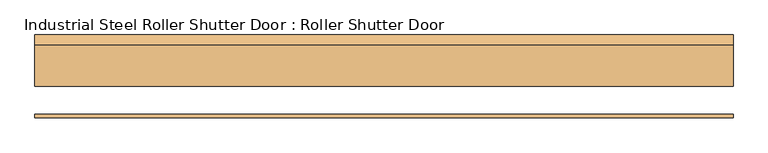
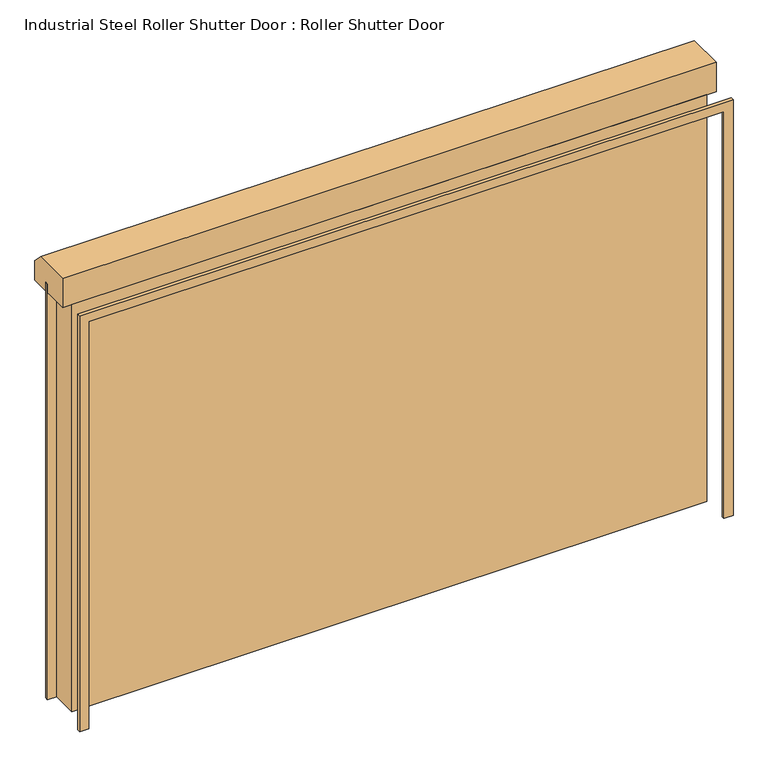
"""IFC4 building model written with IfcOpenShell, lengths in millimetres: door geometry, Industrial Steel Roller Shutter Door : Roller Shutter Door."""

from ifc_helpers import new_model, si_unit, frame, origin, place, context, project, spatial, polyline, outline, extrude, source, transform, mapped, element, save


def industrial_steel_roller_shutter_door_roller_shutter_door_28cb9aac(model_context):
    return source(origin(), model_context, "Body", "SweptSolid", [
        extrude(outline(polyline([(3500.0, -2580.0), (3500.0, 2580.0), (0.0, 2580.0), (0.0, 2655.0), (3575.0, 2655.0), (3575.0, -2655.0), (0.0, -2655.0), (0.0, -2580.0), (3500.0, -2580.0)])), frame((0.0, 215.0, 0.0), z_axis=(0.0, 1.0, 0.0), x_axis=(0.0, 0.0, 1.0)), (0.0, 0.0, 1.0), 25.0),
        extrude(outline(polyline([(3575.0, -2655.0), (0.0, -2655.0), (0.0, -2580.0), (3500.0, -2580.0), (3500.0, 2580.0), (0.0, 2580.0), (0.0, 2655.0), (3575.0, 2655.0), (3575.0, -2655.0)])), frame((0.0, -240.0, 0.0), z_axis=(0.0, 1.0, 0.0), x_axis=(0.0, 0.0, 1.0)), (0.0, 0.0, 1.0), 25.0),
        extrude(outline(polyline([(0.0, 3500.0), (215.0, 3500.0), (215.0, 3475.0), (240.0, 3475.0), (240.0, 0.0), (0.0, 0.0), (0.0, 3500.0)])), frame((-2580.0, 0.0, 0.0), z_axis=(1.0, 0.0, 0.0), x_axis=(0.0, 1.0, 0.0)), (0.0, 0.0, 1.0), 5160.0),
        extrude(outline(polyline([(0.0, 3750.0), (310.0, 3750.0), (390.0, 3670.0), (390.0, 3500.0), (0.0, 3500.0), (0.0, 3750.0)])), frame((-2655.0, 0.0, 0.0), z_axis=(1.0, 0.0, 0.0), x_axis=(0.0, 1.0, 0.0)), (0.0, 0.0, 1.0), 5310.0),
    ])


if __name__ == "__main__":
    model = new_model("IFC4")
    model_context = context("Model", 3, world=origin())
    ifc_project = project(units=[si_unit("LENGTHUNIT", "METRE", prefix="MILLI")], contexts=[model_context])
    site = spatial("IfcSite", under=ifc_project)
    building = spatial("IfcBuilding", under=site)
    placement = place(None, origin())
    industrial_steel_roller_shutter_door_roller_shutter_door_shape = industrial_steel_roller_shutter_door_roller_shutter_door_28cb9aac(model_context)
    element("IfcDoor", 1, ObjectType="Industrial Steel Roller Shutter Door : Roller Shutter Door", at=placement, inside=building, context=model_context, shape_type="MappedRepresentation", body=[
        mapped(industrial_steel_roller_shutter_door_roller_shutter_door_shape, transform((0.0, 0.0, 0.0), x_axis=(1.0, 0.0, 0.0), y_axis=(0.0, 1.0, 0.0), z_axis=(0.0, 0.0, 1.0))),
    ])
    save(model, "model.ifc")

# Revit data of these elements
# Type "Industrial Steel Roller Shutter Door : Roller Shutter Door"
#   Description = "External Roller Shutter Door"
#   Type Mark = "52"
#   Frame Projection Ext. = 25 mm
#   Frame Projection Int. = 25 mm
#   Frame Width = 75 mm
#   Height = 3500 mm
#   Width = 5160 mm
#   Function = (empty or 0)
#   Wall Closure = (empty or 0)
#   Assembly Code = ""
# Element 1 (IfcDoor, "Industrial Steel Roller Shutter Door : Roller Shutter Door")
#   Materials on its faces: "Steel Shutters", "Render 0-255-0"
# Materials
#   "Steel Shutters": class "Vinyl", colour RGB 122 127 125, transparency 0
#   "Render 0-255-0": class "Miscellaneous", colour RGB 0 255 0, transparency 0
